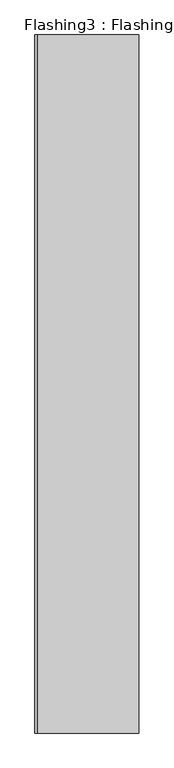
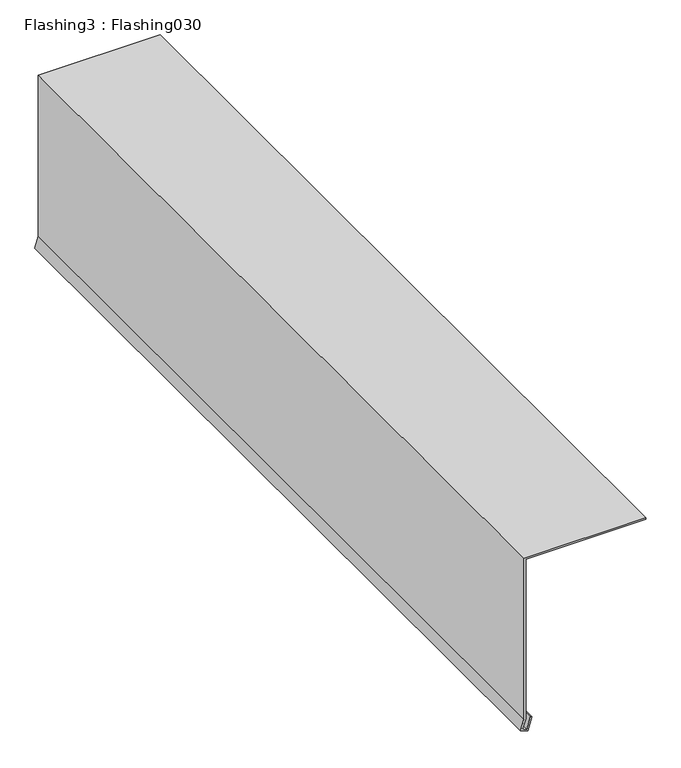
"""IFC4 building model written with IfcOpenShell, lengths in millimetres: proxy geometry, Flashing3 : Flashing030."""

import ifcopenshell
import ifcopenshell.guid

model = None  # the IFC model being written
_history = None  # IfcOwnerHistory: only IFC2X3 demands one
_inside = {}  # id of a spatial element -> (the spatial element, [elements in it])
_under = {}  # id of a project, library or spatial element -> (it, [spatial elements below it])
_declared = {}  # id of a project -> (the project, [libraries it declares])
_typed = {}  # id of a type object -> (the type object, [elements of that type])
_made_of = {}  # id of a material, layer set ... -> (it, [elements and type objects made of it])


def new_model(schema):
    """Start an empty IFC model of exactly this schema.

    Asked for "IFC4X3", IfcOpenShell would pick the latest addendum, in which some entities
    have other attributes; the version numbers below select the first issue.
    IFC2X3 requires an IfcOwnerHistory on every rooted entity: one is made here for all.
    """
    global model, _history
    if schema == "IFC4X3":
        model = ifcopenshell.file(schema_version=(4, 3, 0, 0))
    else:
        model = ifcopenshell.file(schema=schema)
    _inside.clear()
    _under.clear()
    _declared.clear()
    _typed.clear()
    _made_of.clear()
    _history = None
    if model.schema == "IFC2X3":
        org = make("IfcOrganization", Name="unknown")
        user = make(
            "IfcPersonAndOrganization",
            ThePerson=make("IfcPerson", FamilyName="unknown"),
            TheOrganization=org,
        )
        app = make(
            "IfcApplication",
            ApplicationDeveloper=org,
            Version="unknown",
            ApplicationFullName="unknown",
            ApplicationIdentifier="unknown",
        )
        _history = make(
            "IfcOwnerHistory",
            OwningUser=user,
            OwningApplication=app,
            ChangeAction="ADDED",
            CreationDate=0,
        )
    return model


def make(cls, **values):
    """One entity of the class cls with the attributes given. An attribute that is None is left unset."""
    return model.create_entity(
        cls, **{name: value for name, value in values.items() if value is not None}
    )


def rooted(cls, **values):
    """An entity with a GlobalId (a new one), such as an element, a storey or a relation."""
    return make(cls, GlobalId=ifcopenshell.guid.new(), OwnerHistory=_history, **values)


def si_unit(unit_type, name, prefix=None):
    """IfcSIUnit, for example si_unit("LENGTHUNIT", "METRE", prefix="MILLI")."""
    return make("IfcSIUnit", UnitType=unit_type, Prefix=prefix, Name=name)


def assignment(units):
    """IfcUnitAssignment: the units of a project."""
    return None if units is None else make("IfcUnitAssignment", Units=units)


def point(xyz):
    """IfcCartesianPoint."""
    return None if xyz is None else make("IfcCartesianPoint", Coordinates=xyz)


def direction(xyz):
    """IfcDirection."""
    return None if xyz is None else make("IfcDirection", DirectionRatios=xyz)


def frame(location, z_axis=None, x_axis=None):
    """IfcAxis2Placement3D, a coordinate frame: its origin and axes. An axis left out is left unset."""
    return make(
        "IfcAxis2Placement3D",
        Location=point(location),
        Axis=direction(z_axis),
        RefDirection=direction(x_axis),
    )


def origin():
    """The frame at (0, 0, 0) with its axes left unset."""
    return frame((0.0, 0.0, 0.0))


def place(relative_to, where):
    """IfcLocalPlacement: puts the frame where relative to a parent placement (None: the world)."""
    return make(
        "IfcLocalPlacement", PlacementRelTo=relative_to, RelativePlacement=where
    )


def context(
    kind, dimensions, precision=None, world=None, true_north=None, identifier=None
):
    """IfcGeometricRepresentationContext, for example the 3D "Model" context."""
    return make(
        "IfcGeometricRepresentationContext",
        ContextIdentifier=identifier,
        ContextType=kind,
        CoordinateSpaceDimension=dimensions,
        Precision=precision,
        WorldCoordinateSystem=world,
        TrueNorth=true_north,
    )


def project(units=None, contexts=None):
    """IfcProject with its units and contexts."""
    return rooted(
        "IfcProject",
        Name="project",
        RepresentationContexts=contexts,
        UnitsInContext=assignment(units),
    )


def spatial(cls, under=None, at=None, **own):
    """A site, building, storey or space (cls), placed at a placement, below another one or the project."""
    s = rooted(cls, ObjectPlacement=at, **own)
    if under is not None:
        _under.setdefault(under.id(), (under, []))[1].append(s)
    return s


def polyline(points):
    """IfcPolyline through the points."""
    return make("IfcPolyline", Points=[point(p) for p in points])


def outline(outer, holes=None, kind="AREA"):
    """IfcArbitraryClosedProfileDef: a profile drawn as a closed curve; with holes, ...WithVoids."""
    if holes is None:
        return make("IfcArbitraryClosedProfileDef", ProfileType=kind, OuterCurve=outer)
    return make(
        "IfcArbitraryProfileDefWithVoids",
        ProfileType=kind,
        OuterCurve=outer,
        InnerCurves=holes,
    )


def extrude(swept, where, along, depth):
    """IfcExtrudedAreaSolid: the profile swept, set in the frame where, extruded along a direction by depth."""
    return make(
        "IfcExtrudedAreaSolid",
        SweptArea=swept,
        Position=where,
        ExtrudedDirection=direction(along),
        Depth=depth,
    )


def shape(context_of_items, identifier, shape_type, items):
    """IfcShapeRepresentation: the items that make up one representation, for example the "Body"."""
    return make(
        "IfcShapeRepresentation",
        ContextOfItems=context_of_items,
        RepresentationIdentifier=identifier,
        RepresentationType=shape_type,
        Items=items,
    )


def source(mapping_origin, context_of_items, identifier, shape_type, items):
    """IfcRepresentationMap: a shape defined once, which mapped items show again and again."""
    return make(
        "IfcRepresentationMap",
        MappingOrigin=mapping_origin,
        MappedRepresentation=shape(context_of_items, identifier, shape_type, items),
    )


def transform(
    local_origin,
    x_axis=None,
    y_axis=None,
    z_axis=None,
    scale=None,
    scale2=None,
    scale3=None,
    uniform=True,
):
    """IfcCartesianTransformationOperator3D, or its non-uniform kind. x_axis, y_axis, z_axis: its Axis1, 2, 3."""
    if uniform:
        return make(
            "IfcCartesianTransformationOperator3D",
            Axis1=direction(x_axis),
            Axis2=direction(y_axis),
            LocalOrigin=point(local_origin),
            Scale=scale,
            Axis3=direction(z_axis),
        )
    return make(
        "IfcCartesianTransformationOperator3DnonUniform",
        Axis1=direction(x_axis),
        Axis2=direction(y_axis),
        LocalOrigin=point(local_origin),
        Scale=scale,
        Axis3=direction(z_axis),
        Scale2=scale2,
        Scale3=scale3,
    )


def mapped(mapping_source, mapping_target):
    """IfcMappedItem: shows the shape of a source again, moved by a transform."""
    return make(
        "IfcMappedItem", MappingSource=mapping_source, MappingTarget=mapping_target
    )


def made_of(thing, what):
    """Note that an element or type object is made of a material, layer set ...; save() writes the relation."""
    if what is not None:
        _made_of.setdefault(what.id(), (what, []))[1].append(thing)
    return thing


def element(
    cls,
    number,
    at=None,
    inside=None,
    cuts=None,
    type_object=None,
    material=None,
    context=None,
    identifier="Body",
    shape_type=None,
    held_by="IfcProductDefinitionShape",
    body=None,
    shapes=None,
    **own,
):
    """One element of the class cls, such as IfcWall. Its Tag is "e" and its number.

    at: its placement. inside: the storey or other place that contains it. cuts: it is an
    opening in that element (IfcRelVoidsElement). A single representation is given by context,
    identifier, shape_type and body (its items); several are given by shapes. held_by: the class
    of the entity that holds the representations. save() writes the other relations.
    """
    e = rooted(cls, Tag="e%d" % number, ObjectPlacement=at, **own)
    if body is not None:
        shapes = [shape(context, identifier, shape_type, body)]
    if shapes is not None:
        e.Representation = make(held_by, Representations=shapes)
    if inside is not None:
        _inside.setdefault(inside.id(), (inside, []))[1].append(e)
    if cuts is not None:
        rooted(
            "IfcRelVoidsElement", RelatingBuildingElement=cuts, RelatedOpeningElement=e
        )
    if type_object is not None:
        _typed.setdefault(type_object.id(), (type_object, []))[1].append(e)
    return made_of(e, material)


def aggregate(whole, parts):
    """IfcRelAggregates: a whole, such as a stair, and the parts it consists of."""
    return rooted("IfcRelAggregates", RelatingObject=whole, RelatedObjects=parts)


def save(model, path):
    """Write the relations noted so far, then the file.

    IfcRelAggregates (storeys below a building ...), IfcRelContainedInSpatialStructure (elements
    in a storey), IfcRelDefinesByType, IfcRelAssociatesMaterial and IfcRelDeclares: one each for
    every whole, place, type object, material and project.
    """
    for whole, parts in _under.values():
        aggregate(whole, parts)
    for where, things in _inside.values():
        rooted(
            "IfcRelContainedInSpatialStructure",
            RelatedElements=things,
            RelatingStructure=where,
        )
    for kind, things in _typed.values():
        rooted("IfcRelDefinesByType", RelatedObjects=things, RelatingType=kind)
    for what, things in _made_of.values():
        rooted("IfcRelAssociatesMaterial", RelatedObjects=things, RelatingMaterial=what)
    for by, libraries in _declared.values():
        rooted("IfcRelDeclares", RelatingContext=by, RelatedDefinitions=libraries)
    model.write(path)


def flashing3_flashing030_6e34a50e(model_context):
    return source(origin(), model_context, "Body", "SweptSolid", [
        extrude(outline(polyline([(43752.7647284, 5308.7501869), (43725.7732624, 5300.464438), (43720.3821423, 5318.0264272), (43751.7544661, 5327.7395586), (43752.9374956, 5323.9185062), (43725.3718611, 5315.3839573), (43728.4045857, 5305.4564195), (43752.1645952, 5312.7501869), (44153.1848954, 5312.7501869), (44153.1848954, 5598.5706647), (44157.1848954, 5598.5706647), (44157.1848954, 5308.7501869), (43752.7647284, 5308.7501869)])), frame((0.0, -1052.8906574, 0.0), z_axis=(0.0, 1.0, 0.0), x_axis=(0.0, 0.0, 1.0)), (0.0, 0.0, 1.0), 1999.85),
    ])


if __name__ == "__main__":
    model = new_model("IFC4")
    model_context = context("Model", 3, world=origin())
    ifc_project = project(units=[si_unit("LENGTHUNIT", "METRE", prefix="MILLI")], contexts=[model_context])
    site = spatial("IfcSite", under=ifc_project)
    building = spatial("IfcBuilding", under=site)
    placement = place(None, origin())
    flashing3_flashing030_shape = flashing3_flashing030_6e34a50e(model_context)
    element("IfcBuildingElementProxy", 1, Name="Flashing3 : Flashing030", ObjectType="Flashing3 : Flashing030", at=placement, inside=building, context=model_context, shape_type="MappedRepresentation", body=[
        mapped(flashing3_flashing030_shape, transform((0.0, 0.0, 0.0), x_axis=(1.0, 0.0, 0.0), y_axis=(0.0, 1.0, 0.0), z_axis=(0.0, 0.0, 1.0))),
    ])
    save(model, "model.ifc")

# Revit data of these elements
# Type "Flashing3 : Flashing030"
#   NameOverride = "Flashing030"
# Element 1 (IfcBuildingElementProxy, "Flashing3 : Flashing030")
#   Materials on its faces: "BRAKE METAL EAVE TRIM TO MATCH STANDING SEAM COLOR"
# Materials
#   "BRAKE METAL EAVE TRIM TO MATCH STANDING SEAM COLOR": class "Unassigned", colour RGB 128 128 128, transparency 0, Cost = 0
